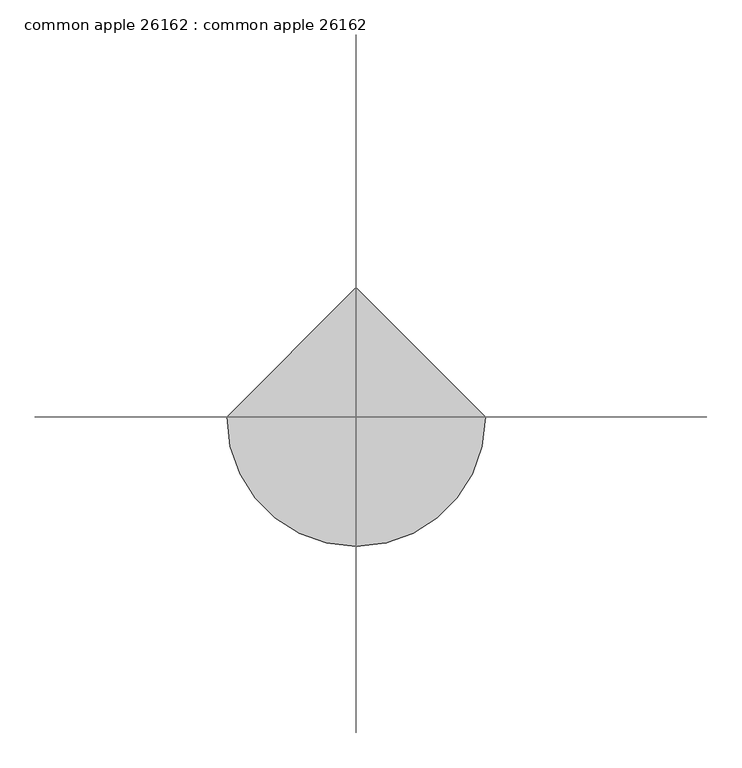
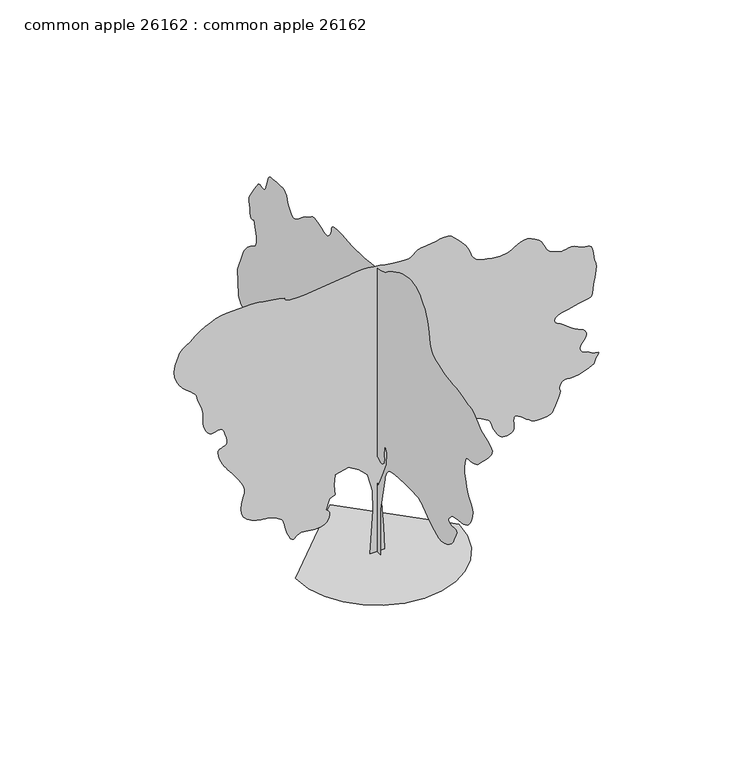
"""IFC4 building model written with IfcOpenShell, lengths in millimetres: proxy geometry, common apple 26162 : common apple 26162."""

from ifc_helpers import new_model, si_unit, origin, place, context, project, spatial, triangles, source, transform, mapped, element, save


def common_apple_26162_common_apple_26162_2cf08d23(model_context):
    return source(origin(), model_context, "Body", "Tessellation", [
        triangles([(-6.61e-05, -106.7031981, 0.0075972), (-6.25e-05, 141.1357166, 0.0075898), (-4.92e-05, 101.4814601, 465.9455781), (-3.19e-05, 131.2220957, 1031.0173004), (-1.83e-05, 230.3576144, 1437.4734501), (-8.7e-06, 398.8869896, 1675.3980263), (-1.1e-06, 587.2459139, 1834.016106), (2.7e-06, 765.6887283, 1873.6680462), (3.6e-06, 963.961219, 1804.2751888), (1.5e-06, 1023.4430534, 1705.1389435), (-4.1e-06, 904.4794573, 1576.2617809), (-8.5e-06, 944.1340136, 1407.7326782), (-1.46e-05, 1172.144878, 1090.4990622), (-1.49e-05, 1568.687534, 882.3128597), (-8.7e-06, 2143.6727863, 803.006436), (7.7e-06, 2490.6473923, 1179.7191977), (2.57e-05, 2847.5453751, 1606.0026981), (3.25e-05, 3402.6882339, 1556.4345028), (3.9e-05, 3600.9610153, 1675.3980263), (4.6e-05, 3591.0549339, 1913.3226025), (4.57e-05, 3412.6196045, 1992.6315697), (5.03e-05, 3283.7399712, 2210.7288677), (5.51e-05, 3591.0549339, 2220.6425068), (6.07e-05, 4205.6845688, 2101.6814541), (6.29e-05, 4275.3567696, 2137.8384041), (6.49e-05, 4342.3114037, 2174.2544952), (6.7e-05, 4403.9061905, 2211.1911942), (6.89e-05, 4457.4241447, 2248.9101128), (7.07e-05, 4500.1976967, 2287.6680668), (7.23e-05, 4529.5348595, 2327.7263775), (7.37e-05, 4542.7427742, 2369.3469475), (8.93e-05, 4572.4863075, 2874.9268433), (9.94e-05, 4403.9570595, 3301.215358), (0.0001002, 4386.5834106, 3334.8449913), (0.000101, 4360.9041641, 3374.6975006), (0.0001018, 4328.265168, 3418.5378479), (0.0001026, 4290.0887192, 3464.105706), (0.0001033, 4247.7471176, 3509.1651649), (0.0001039, 4202.636499, 3551.4561882), (0.0001043, 4156.1291634, 3588.718158), (0.0001045, 4111.323468, 3617.9027138), (0.0001046, 4070.8611122, 3640.1530998), (0.0001046, 4035.4281006, 3659.4571541), (0.0001048, 4005.7101471, 3679.8024239), (0.0001052, 3982.4182549, 3705.2026176), (0.000106, 3966.2384285, 3739.5941231), (0.0001073, 3957.8566727, 3786.9906487), (0.0001089, 3956.7898773, 3842.7945099), (0.0001107, 3961.4378494, 3899.6395866), (0.0001126, 3970.8614021, 3957.3738533), (0.0001145, 3984.0948967, 4015.7685448), (0.0001165, 4000.1982742, 4074.6966339), (0.0001185, 4018.2070587, 4133.9802246), (0.0001206, 4037.1553207, 4193.4417114), (0.0001203, 4062.5299347, 4172.9947037), (0.0001202, 4087.2188347, 4157.4244331), (0.0001204, 4110.5107269, 4151.5570587), (0.000121, 4131.7196068, 4160.2693176), (0.0001221, 4150.160051, 4188.3870781), (0.0001239, 4165.1460548, 4240.787368), (0.0001265, 4175.9410355, 4322.3213448), (0.000129, 4186.6092796, 4402.5600517), (0.0001308, 4198.1408432, 4455.5698975), (0.000132, 4205.3543564, 4492.9588943), (0.000133, 4202.9922913, 4526.3597626), (0.0001339, 4185.923275, 4567.406385), (0.0001352, 4148.8900703, 4627.7059021), (0.000137, 4086.736306, 4718.8666168), (0.0001389, 4019.8834099, 4816.9867905), (0.0001404, 3969.4896835, 4892.043837), (0.0001414, 3931.4405525, 4946.4759796), (0.0001421, 3901.5194138, 4982.6714447), (0.0001423, 3875.5858223, 5003.1184525), (0.0001421, 3849.5002052, 5010.2046478), (0.0001416, 3819.0709579, 5006.343837), (0.0001408, 3787.3208611, 4996.7176804), (0.0001401, 3759.4062859, 4987.6240494), (0.0001396, 3734.2601463, 4983.2045517), (0.0001394, 3710.841227, 4987.6240494), (0.0001396, 3688.1338921, 5005.0485672), (0.0001402, 3665.0704742, 5039.6435486), (0.0001416, 3640.6103394, 5095.574437), (0.0001432, 3619.2235634, 5160.9030075), (0.0001447, 3603.043737, 5219.9581238), (0.000146, 3587.5496246, 5271.4183548), (0.000147, 3568.2455704, 5313.8366959), (0.0001475, 3540.6103386, 5345.8661362), (0.0001475, 3500.1482735, 5366.109668), (0.0001469, 3442.3378487, 5373.1458664), (0.0001459, 3372.4368828, 5376.2445145), (0.0001451, 3300.6055115, 5383.3312912), (0.0001442, 3229.8412262, 5391.1034912), (0.0001434, 3163.0391991, 5396.2851517), (0.0001425, 3103.1713417, 5395.5485687), (0.0001414, 3053.2095657, 5385.642778), (0.0001402, 3016.0746231, 5363.2394943), (0.0001391, 2991.8429626, 5337.2044556), (0.0001382, 2976.4758774, 5316.3510773), (0.0001375, 2966.6462448, 5297.4283951), (0.0001368, 2959.0769394, 5277.1081238), (0.0001359, 2950.4664185, 5252.1148819), (0.0001348, 2937.5122673, 5219.1198029), (0.0001331, 2916.9382324, 5174.873085), (0.0001313, 2890.1666107, 5126.1051315), (0.0001296, 2860.6265533, 5083.2042618), (0.000128, 2827.9619774, 5048.4569641), (0.0001268, 2791.8432518, 5024.124147), (0.0001258, 2751.8890045, 5012.4399765), (0.0001253, 2707.794603, 5015.6909409), (0.0001252, 2659.1789658, 5036.0873703), (0.0001254, 2610.791803, 5068.0662323), (0.0001258, 2565.8846603, 5103.6768494), (0.0001263, 2521.8332794, 5141.7006912), (0.0001267, 2476.0523529, 5180.9436447), (0.0001272, 2425.9356445, 5220.212178), (0.0001274, 2368.8821503, 5258.2360199), (0.0001275, 2302.2908661, 5293.846637), (0.0001276, 2240.2945049, 5328.4671982), (0.0001279, 2193.5584042, 5362.0459625), (0.0001282, 2154.2798424, 5391.129071), (0.0001282, 2114.6558075, 5412.2365036), (0.0001278, 2066.8783459, 5421.8882401), (0.0001267, 2003.1496777, 5416.6304214), (0.0001247, 1915.6618492, 5392.9830276), (0.0001224, 1826.1497257, 5361.2837997), (0.0001207, 1757.9710384, 5335.9853439), (0.0001194, 1705.7434124, 5319.8816757), (0.0001187, 1664.0950825, 5315.7418121), (0.0001184, 1627.6484699, 5326.358606), (0.0001187, 1591.0293388, 5354.4766571), (0.0001195, 1548.8602558, 5402.8893997), (0.0001207, 1514.8419834, 5459.7853455), (0.000122, 1498.8602554, 5510.7630478), (0.0001232, 1489.8128426, 5554.806871), (0.0001241, 1476.6047825, 5590.874437), (0.0001244, 1448.1338459, 5617.9256927), (0.0001241, 1393.3079773, 5634.9182602), (0.0001229, 1301.0220406, 5640.8109238), (0.0001214, 1201.3955635, 5639.6935501), (0.0001202, 1126.7398006, 5636.6454803), (0.0001192, 1069.2519579, 5632.2259827), (0.0001184, 1021.1290958, 5626.9425842), (0.0001175, 974.5682751, 5621.3039749), (0.0001165, 921.7642307, 5615.8426804), (0.0001154, 854.9113346, 5611.0679718), (0.0001143, 784.7082069, 5608.019902), (0.0001133, 723.0014357, 5607.2071609), (0.0001125, 663.7228592, 5608.4768509), (0.0001116, 600.8019178, 5611.6516571), (0.0001107, 528.1680156, 5616.5792633), (0.0001096, 439.7556433, 5623.0567749), (0.0001082, 329.4941322, 5630.9051331), (0.0001067, 206.9466705, 5641.7254028), (0.0001053, 88.3885184, 5656.6861176), (0.0001042, -22.1921751, 5675.1262711), (0.0001034, -120.8075788, 5696.3354416), (0.0001029, -203.4686488, 5719.6276245), (0.0001027, -266.1871316, 5744.3162338), (0.0001028, -304.9729546, 5769.6908478), (0.0001032, -347.9523442, 5804.4381454), (0.0001036, -420.583703, 5853.4089935), (0.0001039, -514.8939712, 5910.1532043), (0.000104, -622.9024584, 5968.31884), (0.0001039, -736.6335978, 6021.4301331), (0.0001035, -848.1092062, 6063.1118912), (0.0001027, -949.3562239, 6086.9371811), (0.0001016, -1039.2697763, 6095.8017563), (0.0001004, -1122.4243664, 6096.0046509), (9.9e-05, -1199.3330441, 6086.1494385), (9.73e-05, -1270.5191059, 6064.8391113), (9.53e-05, -1336.5033051, 6030.7016602), (9.29e-05, -1397.8062492, 5982.3650757), (9.01e-05, -1454.9462208, 5918.407933), (8.77e-05, -1502.3755932, 5861.1056168), (8.62e-05, -1536.9730453, 5825.4944183), (8.5e-05, -1562.8963177, 5799.256485), (8.38e-05, -1584.313615, 5770.0716385), (8.22e-05, -1605.3828232, 5725.6220261), (7.96e-05, -1630.2698215, 5653.5874695), (7.58e-05, -1663.1323505, 5541.6751144), (7.16e-05, -1693.8258259, 5415.6147858), (6.81e-05, -1715.6747829, 5307.5626602), (6.5e-05, -1738.0446384, 5214.9799393), (6.21e-05, -1770.3000824, 5135.1981812), (5.93e-05, -1821.8062408, 5065.6530075), (5.62e-05, -1901.9230076, 5003.7532974), (5.28e-05, -2020.0178341, 4946.8823502), (4.95e-05, -2152.913356, 4902.7117905), (4.69e-05, -2273.494804, 4876.3974083), (4.48e-05, -2385.2295536, 4861.5384315), (4.29e-05, -2491.5921021, 4851.7340881), (4.1e-05, -2596.0345642, 4840.5071571), (3.89e-05, -2702.0542557, 4821.482737), (3.62e-05, -2813.1030006, 4788.2594742), (3.39e-05, -2912.3155495, 4758.5159409), (3.24e-05, -2986.585144, 4746.9843773), (3.14e-05, -3044.8780975, 4742.742485), (3.04e-05, -3096.2371719, 4734.8432579), (2.89e-05, -3149.6786774, 4712.3896866), (2.66e-05, -3214.2200867, 4664.4344742), (2.28e-05, -3298.878582, 4580.0809021), (1.85e-05, -3408.6320572, 4492.8062874), (1.5e-05, -3530.0185432, 4434.3354378), (1.2e-05, -3644.3188339, 4390.95233), (9.4e-06, -3732.7616913, 4348.9659393), (7.2e-06, -3776.6273277, 4294.6608238), (5.1e-06, -3757.196537, 4214.3459587), (3e-06, -3655.7486595, 4094.3056114), (1.1e-06, -3529.027906, 3968.7786804), (-3e-07, -3439.3912262, 3876.7287758), (-1.3e-06, -3376.6531952, 3811.5525215), (-1.9e-06, -3330.5522301, 3766.670668), (-2.3e-06, -3290.852037, 3735.479258), (-2.3e-06, -3247.3671913, 3711.4002045), (-2.2e-06, -3189.8108208, 3687.854258), (-1.7e-06, -3124.3802216, 3671.1919029), (-1e-06, -3064.487075, 3666.3404549), (-2e-07, -3010.8420937, 3664.4356293), (2e-07, -2964.1568619, 3656.6378494), (2e-07, -2925.0662247, 3634.0825401), (-8e-07, -2894.3070557, 3587.9559952), (-2.8e-06, -2872.5897766, 3509.3939301), (-5.1e-06, -2860.8041588, 3423.8465355), (-7.1e-06, -2858.3659355, 3357.9081184), (-8.8e-06, -2863.7507813, 3304.4410332), (-1.04e-05, -2875.358503, 3256.3335045), (-1.21e-05, -2891.6653564, 3206.498465), (-1.41e-05, -2911.070858, 3147.8244301), (-1.67e-05, -2932.0768433, 3073.199334), (-1.95e-05, -2961.2613991, 2993.8242371), (-2.22e-05, -3001.7234642, 2923.6186386), (-2.47e-05, -3046.5291595, 2859.6612053), (-2.72e-05, -3088.7187355, 2798.9806068), (-2.95e-05, -3121.3830208, 2738.6555099), (-3.16e-05, -3137.5628471, 2675.7398735), (-3.35e-05, -3130.349334, 2607.2612045), (-3.52e-05, -3109.3942177, 2540.281572), (-3.66e-05, -3087.7280983, 2482.819091), (-3.77e-05, -3063.4964378, 2433.5098915), (-3.85e-05, -3034.7182526, 2390.964814), (-3.91e-05, -2999.5645844, 2353.7970245), (-3.94e-05, -2956.0544495, 2320.6169277), (-3.96e-05, -2902.3333099, 2290.0378349), (-3.93e-05, -2836.3948929, 2266.2507694), (-3.86e-05, -2760.9314758, 2251.4832115), (-3.77e-05, -2680.9721123, 2241.3942924), (-3.68e-05, -2601.4955681, 2231.6559334), (-3.61e-05, -2527.6041481, 2217.9272655), (-3.58e-05, -2464.279525, 2195.8749779), (-3.62e-05, -2416.56049, 2161.1632885), (-3.68e-05, -2383.2356346, 2123.2410393), (-3.73e-05, -2359.9691769, 2093.2995529), (-3.79e-05, -2347.1065899, 2069.598674), (-3.84e-05, -2344.9984337, 2050.4090023), (-3.9e-05, -2353.9875652, 2033.9929985), (-3.98e-05, -2374.4217831, 2018.6158848), (-4.07e-05, -2406.646851, 2002.5452087), (-4.16e-05, -2449.8269188, 1993.9041664), (-4.23e-05, -2498.3841293, 1996.5330757), (-4.28e-05, -2545.5646797, 2002.2862129), (-4.34e-05, -2584.5791588, 2003.0075352), (-4.41e-05, -2608.6837921, 1990.5513187), (-4.52e-05, -2611.0967262, 1956.7642822), (-4.66e-05, -2585.0869766, 1893.4953243), (-4.83e-05, -2549.9080193, 1821.1814243), (-4.96e-05, -2524.6272949, 1762.91376), (-5.07e-05, -2502.1126808, 1714.5318295), (-5.16e-05, -2475.2625755, 1671.8725147), (-5.23e-05, -2436.9668026, 1630.7726978), (-5.27e-05, -2380.1140228, 1587.0720222), (-5.3e-05, -2297.5969666, 1536.6072247), (-5.28e-05, -2203.8378639, 1496.8968578), (-5.19e-05, -2116.842738, 1484.7582092), (-5.03e-05, -2034.8743401, 1494.9892708), (-4.83e-05, -1956.2028339, 1522.3883251), (-4.6e-05, -1879.090971, 1561.7532188), (-4.35e-05, -1801.803828, 1607.8822346), (-4.09e-05, -1722.6115688, 1655.5707481), (-3.83e-05, -1647.9584221, 1703.6352562), (-3.59e-05, -1583.013113, 1752.3931812), (-3.37e-05, -1524.1383636, 1798.8980461), (-3.16e-05, -1467.6919544, 1840.2010483), (-2.97e-05, -1410.0313751, 1873.3506237), (-2.82e-05, -1347.5167316, 1895.4053822), (-2.69e-05, -1276.503479, 1903.4089634), (-2.54e-05, -1177.6846561, 1904.2776604), (-2.33e-05, -1044.3574018, 1905.4916851), (-2.11e-05, -891.7820492, 1904.9710773), (-1.89e-05, -735.2163151, 1900.6352955), (-1.7e-05, -589.9230761, 1890.4040886), (-1.58e-05, -471.1627742, 1872.1948803), (-1.55e-05, -394.1956335, 1843.9297451), (-1.6e-05, -348.7041879, 1805.3140789), (-1.68e-05, -313.0958962, 1758.377409), (-1.8e-05, -285.7248199, 1704.5039532), (-1.95e-05, -264.9450744, 1645.0805454), (-2.11e-05, -249.1058704, 1581.494165), (-2.29e-05, -236.5620685, 1515.1341167), (-2.48e-05, -225.6659676, 1447.3870892), (-3.91e-05, -116.6168281, 912.0537769), (-2.05e-05, -27.3946828, 1318.5099266), (-1.32e-05, -176.0980811, 1635.74347), (-6.6e-06, -304.975498, 1923.2362415), (2e-07, -324.8002327, 2161.1632885), (4.8e-06, -255.4073572, 2280.1241959), (-4e-07, -225.6657133, 2091.767815), (-1.7e-06, -231.7353101, 2049.4539734), (-3e-06, -235.984215, 2008.1814926), (-4.2e-06, -236.5910275, 1968.9892628), (-5.2e-06, -231.7353101, 1932.9186447), (-6e-06, -219.5961346, 1901.0111446), (-6.5e-06, -198.3530817, 1874.3056526), (-6.6e-06, -166.1844602, 1853.8433842), (-6.2e-06, -129.2182845, 1848.5829494), (-5.3e-06, -95.0268123, 1860.3152275), (-4.3e-06, -63.9562343, 1879.3348515), (-3.4e-06, -36.354542, 1895.9235191), (-2.9e-06, -12.5678035, 1900.3761543), (-3.1e-06, 7.0569383, 1882.9772163), (-4.4e-06, 22.1729471, 1834.016106), (-6.1e-06, 32.8958209, 1768.9260384), (-7.8e-06, 39.9768386, 1709.0403042), (-9.4e-06, 44.0233167, 1653.4904972), (-1.1e-05, 45.6418044, 1601.4077751), (-1.24e-05, 45.4396183, 1551.9260571), (-1.39e-05, 44.0233167, 1504.1789715), (-1.53e-05, 41.9999482, 1457.3007282), (139.590126, 0.0003305, 0.0), (-135.4471285, 0.0003387, 0.0), (-74.3278259, 0.000241, 845.4879272), (-84.5142454, 0.0002472, 1242.76455), (-186.3807747, 0.0002013, 1599.294532), (-339.1791879, 0.0002082, 1752.0933449), (-542.9102117, 0.000216, 1874.3335579), (-797.5758808, 0.0002227, 1813.2134514), (-817.9492012, 0.0002203, 1609.4824276), (-797.5758808, 0.0002168, 1415.9368286), (-899.4426281, 0.0002191, 1365.0021469), (-970.7481594, 0.0002183, 1171.4565479), (-951.3247084, 0.0002718, 1158.1240768), (-933.2373676, 0.000271, 1143.3616058), (-917.8246456, 0.0002703, 1125.7517796), (-906.4200365, 0.0002696, 1103.8645981), (-900.3621214, 0.000269, 1076.2750757), (-900.9870106, 0.0002686, 1041.555756), (-909.6280529, 0.0002682, 998.2868128), (-928.5764603, 0.0002681, 955.1042742), (-957.6798437, 0.0002684, 921.0098436), (-994.6267164, 0.0002692, 895.1144766), (-1037.0955631, 0.0002701, 876.5217161), (-1082.7698101, 0.0002713, 864.3449158), (-1129.3382612, 0.0002726, 857.6926329), (-1174.4791832, 0.0002739, 855.6733521), (-1218.6700905, 0.0002753, 858.4063974), (-1263.5747623, 0.0002767, 865.0586803), (-1308.6573303, 0.0002782, 873.3161705), (-1353.3816353, 0.0002796, 880.857498), (-1397.217041, 0.000281, 885.3710306), (-1439.6273884, 0.0002823, 884.5404854), (-1480.0769543, 0.0002833, 876.0466724), (-1514.854628, 0.0002841, 857.900905), (-1542.5051205, 0.0002846, 834.4084436), (-1565.8782578, 0.000285, 812.6990856), (-1587.8238659, 0.0002854, 799.9000122), (-1611.1970032, 0.0002862, 803.1359339), (-1638.8473503, 0.0002874, 829.5392641), (-1673.6225533, 0.000235, 886.2346407), (-1706.6171963, 0.0002371, 959.4984827), (-1729.2790398, 0.0002388, 1029.5593225), (-1744.988982, 0.0002402, 1094.4487484), (-1757.1353336, 0.0002415, 1152.2135365), (-1769.1037891, 0.0002426, 1200.8900711), (-1784.2803337, 0.0002436, 1238.5177162), (-1806.0481911, 0.0002446, 1263.1378704), (-1833.1626698, 0.0002457, 1282.7670502), (-1863.3073414, 0.0002469, 1305.4288937), (-1898.2629112, 0.0002483, 1329.1576778), (-1939.8122646, 0.0002499, 1351.9948013), (-1989.7334908, 0.0002517, 1371.9820988), (-2049.8147072, 0.0002537, 1387.1586433), (-2121.8338577, 0.000256, 1395.5635082), (-2205.4938675, 0.0002044, 1404.6210949), (-2294.67854, 0.0002073, 1424.3695988), (-2382.4381542, 0.0002104, 1456.7724174), (-2461.8232796, 0.0002135, 1503.7853909), (-2525.8821602, 0.0002163, 1567.3691551), (-2567.6627495, 0.0002188, 1649.4849277), (-2580.2355286, 0.0002207, 1752.0933449), (-2568.9835991, 0.0002218, 1851.4048702), (-2548.8159348, 0.0002224, 1927.9097935), (-2527.0379036, 0.0002227, 1989.979842), (-2510.9723145, 0.0001688, 2045.9893593), (-2507.9117455, 0.0001695, 2104.3180664), (-2525.1659248, 0.0001711, 2173.3375454), (-2570.0503944, 0.0001737, 2261.4222851), (-2629.7912247, 0.0001769, 2355.7756828), (-2686.3316689, 0.0001798, 2438.7243988), (-2738.9604332, 0.0001825, 2511.3356644), (-2786.9665146, 0.0001849, 2574.6730774), (-2829.6130394, 0.0001327, 2629.841803), (-2866.1890045, 0.0001345, 2677.8478844), (-2896.008696, 0.000136, 2719.8086952), (-2924.6092758, 0.0001376, 2767.4084061), (-2955.1652596, 0.0001394, 2827.2762634), (-2983.4100471, 0.0001412, 2893.0114952), (-3005.0764572, 0.0001428, 2958.2389091), (-3015.8461487, 0.000144, 3016.5062828), (-3011.4772293, 0.0001446, 3061.4137161), (-2987.7028084, 0.0001442, 3086.5342758), (-2951.4823448, 0.0001433, 3098.8532913), (-2915.109565, 0.0001425, 3111.5533882), (-2882.1147766, 0.0001417, 3127.4282913), (-2856.0800285, 0.0001413, 3149.3740448), (-2840.5350471, 0.0001413, 3180.2349518), (-2839.0871704, 0.0001418, 3222.8561874), (-2855.2669968, 0.0001432, 3280.0823456), (-2877.0348541, 9.05e-05, 3338.9342766), (-2892.2240433, 9.16e-05, 3385.5177704), (-2904.1875572, 9.25e-05, 3421.2048363), (-2916.3286766, 9.32e-05, 3447.4686401), (-2932.0259743, 9.4e-05, 3465.705899), (-2954.70802, 9.48e-05, 3477.3389099), (-2987.7028084, 9.59e-05, 3483.8161308), (-3026.4123642, 9.7e-05, 3481.8857254), (-3064.2583099, 9.8e-05, 3472.1066711), (-3101.5455688, 9.9e-05, 3461.6419029), (-3138.6805115, 0.0001, 3457.552327), (-3175.9930595, 0.0001013, 3467.026458), (-3213.8137161, 0.0001029, 3497.1763618), (-3252.5488518, 0.0001049, 3555.1138138), (-3281.1747208, 0.0001068, 3626.7419998), (-3293.239682, 0.0001082, 3695.3474052), (-3295.8558014, 0.0001093, 3764.1307068), (-3296.1351448, 0.0001104, 3836.3175797), (-3301.2406471, 5.74e-05, 3915.0575409), (-3318.2840836, 5.93e-05, 4003.6274254), (-3354.4028091, 6.19e-05, 4105.2020393), (-3391.2836975, 6.43e-05, 4197.0231789), (-3411.2481766, 6.59e-05, 4259.8120789), (-3422.2972115, 6.68e-05, 4301.925206), (-3432.4570564, 6.76e-05, 4331.7448975), (-3449.7545471, 6.85e-05, 4357.6276199), (-3482.1650688, 6.99e-05, 4387.9804184), (-3537.7657448, 7.22e-05, 4431.1606316), (-3609.6985634, 2.09e-05, 4488.5646858), (-3681.631382, 2.41e-05, 4556.1285851), (-3747.3157448, 2.72e-05, 4634.0305161), (-3800.5287758, 3.01e-05, 4722.4480843), (-3835.047599, 3.26e-05, 4821.5588951), (-3844.6231773, 3.45e-05, 4931.5152649), (-3822.9823471, 3.57e-05, 5052.5468307), (-3789.555899, -1.8e-05, 5157.9310959), (-3763.7749146, -1.77e-05, 5228.187854), (-3739.5941231, -1.77e-05, 5274.3902664), (-3710.9682541, -1.81e-05, 5307.5882401), (-3671.8270386, -1.88e-05, 5338.8555176), (-3616.1246246, -1.98e-05, 5379.1652664), (-3537.7657448, -2.13e-05, 5439.6429703), (-3445.4364967, -2.3e-05, 5511.6775269), (-3351.6849518, -2.48e-05, 5578.225209), (-3256.3079247, -2.67e-05, 5637.4326416), (-3159.1783882, -2.89e-05, 5687.5726044), (-3060.0675774, -3.12e-05, 5726.8155579), (-2958.8228851, -3.39e-05, 5753.4348633), (-2855.2669968, -3.68e-05, 5765.6015625), (-2376.4970924, -5.09e-05, 5775.7869873), (-2309.7356152, -5.29e-05, 5773.1197083), (-2232.8167637, -5.53e-05, 5765.6521408), (-2147.4320045, -3.8e-06, 5754.1458664), (-2055.2781818, -6.7e-06, 5739.4392059), (-1958.0469074, -9.9e-06, 5722.3449005), (-1857.4273224, -1.32e-05, 5703.6251129), (-1755.1159801, -1.65e-05, 5684.1181641), (-1751.9080364, -1.69e-05, 5664.6617935), (-1742.5530842, -1.75e-05, 5646.3739563), (-1720.9022255, -1.83e-05, 5630.3970245), (-1680.8107773, -1.97e-05, 5617.9001129), (-1616.1270802, -2.18e-05, 5610.0261749), (-1520.7042709, -2.46e-05, 5607.9437439), (-1388.3981026, -2.85e-05, 5612.8201904), (-614.2181774, -5.02e-05, 5704.4890137), (-538.3076946, -5.24e-05, 5711.4996323), (-472.1990845, 1e-07, 5721.8879517), (-409.4762778, -1.6e-06, 5732.8355392), (-343.7232419, -3.5e-06, 5741.4460602), (-268.5264692, -5.7e-06, 5744.8749207), (-177.4707081, -8.5e-06, 5740.3031067), (-64.1414019, -1.21e-05, 5724.8598633), (54.7118994, -1.59e-05, 5704.3111176), (159.4882483, -1.93e-05, 5686.4296509), (252.3260954, -2.23e-05, 5671.4183578), (335.3640864, -2.49e-05, 5659.4039749), (410.7386644, -2.73e-05, 5650.6155579), (480.5886887, -2.95e-05, 5645.205423), (547.0529457, -3.15e-05, 5643.3764648), (603.2428662, -3.3e-05, 5651.8346695), (646.0698669, -3.4e-05, 5673.6531052), (683.3697704, -3.47e-05, 5703.4983765), (722.9887184, -3.54e-05, 5736.0359253), (772.7625698, -3.64e-05, 5765.8806152), (840.5349592, -3.81e-05, 5787.6996323), (934.1441437, -4.07e-05, 5796.1828354), (1035.6832947, -4.37e-05, 5802.989978), (1124.0372766, -4.61e-05, 5818.3826431), (1202.2337391, -4.82e-05, 5834.6642075), (1273.3004768, -5.01e-05, 5844.1636276), (1340.2726971, -5.22e-05, 5839.2360214), (1406.173035, -5.46e-05, 5812.2103455), (1474.0342999, -3.2e-06, 5755.4161377), (1539.0152172, -6.2e-06, 5686.9627579), (1594.7301304, -8.7e-06, 5628.1366974), (1641.8903332, -1.09e-05, 5576.0666199), (1681.2120609, -1.28e-05, 5527.9335114), (1713.4041367, -1.44e-05, 5480.8671982), (1739.182505, -1.59e-05, 5431.9975067), (1759.2587505, -1.73e-05, 5378.5304214), (1777.3156425, -1.87e-05, 5324.8604416), (1798.9361252, -2e-05, 5277.2604401), (1827.6839344, -2.15e-05, 5235.5281036), (1867.1225155, 3.1e-05, 5199.4855362), (1920.8180752, 2.9e-05, 5169.0060013), (1992.3318787, 2.65e-05, 5143.8342819), (2085.229842, 2.34e-05, 5123.844223), (2181.6306438, 2.03e-05, 5109.4171967), (2262.7075264, 1.78e-05, 5100.6799393), (2330.5991673, 1.57e-05, 5097.123761), (2387.4419186, 1.4e-05, 5098.1905563), (2435.3767834, 1.27e-05, 5103.3722168), (2476.5374977, 1.16e-05, 5112.0844757), (2513.0678261, 1.07e-05, 5123.844223), (2552.2195061, 9.8e-06, 5144.4947067), (2599.1840813, 8.9e-06, 5175.4829315), (2653.1336952, 7.8e-06, 5209.6459625), (2713.1032906, 6.4e-06, 5239.9226028), (2778.2795448, 4.8e-06, 5259.1249191), (2847.697982, 2.7e-06, 5260.1661346), (2920.5196999, 2e-07, 5235.9094757), (2984.2992371, -2.2e-06, 5202.1528152), (3030.2478859, -4e-06, 5176.5747253), (3062.9883293, -5.3e-06, 5154.908606), (3087.1947006, -6.3e-06, 5132.9122742), (3107.4893921, -7.3e-06, 5106.2679703), (3128.4697975, -8.5e-06, 5070.73293), (3154.8094688, -1e-05, 5021.9905563), (3182.8510712, 4.27e-05, 4971.0890121), (3208.2256851, 4.13e-05, 4930.3473129), (3234.4639091, 4e-05, 4897.4289734), (3265.1724998, 3.87e-05, 4870.0475052), (3303.9076355, 3.72e-05, 4845.8667137), (3354.2252037, 3.53e-05, 4822.6004013), (3419.6808014, 3.3e-05, 4797.8859215), (3486.0258797, 3.08e-05, 4782.8237595), (3540.0769409, 2.92e-05, 4784.7032959), (3586.9909378, 2.8e-05, 4795.4729874), (3631.9489494, 2.68e-05, 4807.1571579), (3680.1326363, 2.55e-05, 4811.7036827), (3736.6730804, 2.36e-05, 4801.0863075), (3806.7519424, 2.1e-05, 4767.3299377), (3879.2181587, 1.84e-05, 4732.9890106), (3939.9240463, 1.63e-05, 4718.4346664), (3989.5811897, 1.48e-05, 4712.2626595), (4028.9003014, 1.35e-05, 4703.0678719), (4058.6185455, 1.22e-05, 4679.4204781), (4079.3957657, 6.51e-05, 4629.9412308), (4091.9941246, 6.34e-05, 4543.2253029), (4103.8306114, 6.18e-05, 4454.6301292), (4119.4261711, 6.04e-05, 4397.0481789), (4135.0217308, 5.94e-05, 4355.3161331), (4146.8835068, 5.84e-05, 4314.2950905), (4151.2268463, 5.74e-05, 4258.8467308), (4144.3688347, 5.64e-05, 4173.8330246), (4122.550399, 5.51e-05, 4044.0642014), (4100.096537, 0.000108, 3908.7329269), (4088.8698967, 0.0001069, 3812.0603394), (4081.3767494, 0.0001061, 3746.5791618), (4070.1501091, 0.0001058, 3704.7962471), (4047.6965378, 0.0001061, 3679.2184479), (4006.548468, 0.0001071, 3662.4034859), (3939.1874634, 0.0001089, 3646.8079262), (3844.4708611, 0.0001114, 3628.5706673), (3734.0822502, 0.0001144, 3608.1998177), (3619.7822502, 0.0001175, 3584.781189), (3513.3053192, 0.0001202, 3557.4761696), (3426.4373657, 0.0001224, 3525.3449913), (3370.9384277, 0.0001234, 3487.4990456), (3358.5429634, 0.0001231, 3443.0744316), (3371.5224037, 0.0001222, 3405.6092766), (3386.2799332, 0.0001214, 3384.1972115), (3405.8633308, 0.0001207, 3371.1669022), (3433.2700882, 0.0001197, 3358.8478867), (3471.5476936, 0.0001182, 3339.5694122), (3523.7447983, 0.0001162, 3305.6857246), (3592.8327324, 0.0001133, 3249.5260712), (3669.2870773, 0.0001101, 3189.9884262), (3740.381575, 0.0001074, 3147.3671906), (3804.5419029, 0.000105, 3116.150782), (3860.1425789, 0.0001572, 3090.8014572), (3905.55783, 0.0001555, 3065.8332138), (3939.2383324, 0.000154, 3035.6833099), (3959.558313, 0.0001528, 2994.8654526), (3960.2948959, 0.0001521, 2946.884951), (3941.8038734, 0.0001519, 2899.2852402), (3912.2635254, 0.0001521, 2852.3968231), (3879.8530037, 0.0001524, 2806.5752014), (3852.8020386, 0.0001525, 2762.1758766), (3839.2892006, 0.0001523, 2719.554641), (3847.5189308, 0.0001514, 2679.0672867), (3870.582058, 0.0001503, 2647.1645828), (3896.1598572, 0.0001492, 2627.2256836), (3924.2270393, 0.0001482, 2614.9319572), (3954.7830231, 0.0001472, 2606.0168037), (3987.8286804, 0.000146, 2596.2121696), (4023.3887192, 0.0001447, 2581.2517456), (4061.4378502, 0.0001432, 2556.842189), (4100.7569618, 0.0001417, 2534.5891869), (4137.7648773, 0.0001405, 2524.8203064), (4168.8798386, 0.0001395, 2521.2847664), (4190.5462486, 0.0001388, 2517.7515518), (4199.2329277, 0.0001384, 2507.9803459), (4191.3334099, 0.0001926, 2485.7375175), (4163.2918076, 0.0001928, 2444.7824593), (4135.3263634, 0.0001929, 2399.7888393), (4122.8550316, 0.0001928, 2366.7332989), (4115.1842789, 0.0001927, 2341.3408081), (4101.6461517, 0.0001927, 2319.3343025), (4071.521537, 0.0001933, 2296.4387524), (4014.1430626, 0.0001946, 2268.3717155), (3918.8166138, 0.0001969, 2230.8633945), (3811.1205711, 0.0001996, 2200.6297749), (3722.1443161, 0.0002021, 2191.0666958), (3649.3987564, 0.0002043, 2192.9081532), (3590.3436401, 0.0002062, 2196.8884335), (3542.540744, 0.0002075, 2193.7413872), (3503.4501068, 0.0002084, 2174.1985394), (3470.6079254, 0.0002087, 2128.9966473), (3451.2532928, 0.0002086, 2081.7474964), (3449.1702805, 0.0002083, 2055.3443115), (3456.7142967, 0.0002078, 2039.4564732), (3466.2137169, 0.0002073, 2023.7466763), (3470.0236588, 0.0002068, 1997.8792145), (3460.4480804, 0.0002064, 1951.5191082), (3429.8662262, 0.0002061, 1874.3335579), (3393.2393921, 0.0002059, 1787.376511), (3366.4171921, 0.0002057, 1717.5239433), (3342.9982727, 0.0002056, 1663.1755165), (3316.5315742, 0.0002058, 1622.7259506), (3280.6157433, 0.0002064, 1594.5725819), (3228.850589, 0.0002077, 1577.1101303), (3154.8094688, 0.0002098, 1568.7357868), (3080.6413216, 0.0002119, 1565.2609989), (3027.8349518, 0.0002135, 1564.6361824), (2989.0998161, 0.0002147, 1568.469088), (2957.146534, 0.0002158, 1578.3572926), (2924.6598541, 0.000217, 1595.9086922), (2884.3248161, 0.0002186, 1622.7259506), (2828.8511673, 0.0002209, 1660.4146385), (2768.830703, 0.0002233, 1702.4363468), (2719.1482704, 0.0002253, 1739.6499184), (2678.9146797, 0.000227, 1769.7336926), (2647.2154518, 0.0002282, 1790.3763279), (2623.1869766, 0.0002291, 1799.2561638), (2605.9403549, 0.0002295, 1794.0567719), (2594.5613983, 0.0002295, 1772.4668106), (2588.1350464, 0.0002293, 1744.7273701), (2585.6459541, 0.000229, 1721.445797), (2586.0014557, 0.0002287, 1700.833683), (2588.1350464, 0.0002283, 1681.1130844), (2591.00522, 0.0002279, 1660.5034412), (2593.494603, 0.0002275, 1637.219252), (2594.5613983, 0.0002271, 1609.4824276), (2593.1135216, 0.0002267, 1579.0989624), (2587.906572, 0.0002264, 1549.7873795), (2577.7211472, 0.0002263, 1522.6143288), (2561.2872665, 0.0002264, 1498.6468964), (2537.3884346, 0.0002268, 1478.9568192), (2504.7494385, 0.0002276, 1464.6108925), (2462.1331444, 0.0002288, 1456.6836147), (2418.7144283, 0.00023, 1454.9893867), (2382.9562912, 0.0002312, 1459.35569), (2352.5447754, 0.0002322, 1470.8491745), (2325.1635979, 0.0002333, 1490.5392517), (2298.4935688, 0.0002346, 1519.4951878), (2270.2207306, 0.000236, 1558.7865395), (2238.0288002, 0.0002377, 1609.4824276), (2208.2396301, 0.0002394, 1664.8392231), (2186.8274197, 0.0001866, 1716.8127949), (2170.9397266, 0.0001878, 1764.5088661), (2157.7241089, 0.0001888, 1807.0362122), (2144.3307404, 0.0001897, 1843.5054977), (2127.9070335, 0.0001907, 1873.0254982), (2105.6033077, 0.0001917, 1894.7068783), (2074.6583942, 0.0001929, 1913.6528149), (2035.1589157, 0.0001944, 1935.2732975), (1988.5319653, 0.0001961, 1959.1214058), (1936.2028919, 0.0001981, 1984.7525448), (1879.5964634, 0.0002001, 2011.717178), (1820.1400635, 0.0002023, 2039.5759426), (1759.2587505, 0.0002046, 2067.8791569), (1412.9141933, 0.0002149, 2067.8791569), (1219.3685944, 0.0002173, 1843.7721966), (1214.8270838, 0.000217, 1813.2134514), (1209.2136909, 0.0002167, 1782.6522354), (1201.4616205, 0.0002165, 1752.0933449), (1190.5040045, 0.0002164, 1721.5345997), (1175.2665625, 0.0002164, 1690.9733837), (1154.6874407, 0.0002165, 1660.4146385), (1127.6898153, 0.0002169, 1629.855748), (1103.6638836, 0.0002172, 1604.0163368), (1088.903956, 0.0002174, 1586.5538853), (1077.7076191, 0.0002175, 1575.8629681), (1064.3726046, 0.0002179, 1570.3384506), (1043.1966442, 0.0002185, 1568.3775238), (1008.4798679, 0.0002195, 1568.3775238), (954.5175367, 0.0002211, 1568.7357868), (886.9839409, 0.0002232, 1571.6161343), (817.1339167, 0.0002254, 1579.3072346), (747.6394667, 0.0002276, 1590.3841747), (681.1726662, 0.0002298, 1603.4220417), (620.41075, 0.0002318, 1616.9957771), (568.0206702, 0.0002335, 1629.6755264), (526.6821324, 0.0002349, 1640.0411728), (491.1627162, 0.0002361, 1650.5543392), (454.5739975, 0.0002374, 1664.275304), (417.0937271, 0.0002388, 1680.6684895), (378.9022719, 0.0002402, 1699.2003525), (340.1748393, 0.0001874, 1719.3350246), (301.0918324, 0.0001889, 1740.5414337), (261.828495, 0.0001904, 1762.2813858), (78.4708189, 0.0002443, 1375.1901878), (68.2843994, 0.0002402, 1079.7776962), (119.217278, 0.0002837, 458.3966929), (-1547.0796959, 1.1e-06, 0.0099807), (-1506.1805935, -354.4877738, 0.0099913), (-1389.6986046, -680.02964, 0.010001), (-1206.9607035, -967.2962626, 0.0100095), (-967.2962626, -1206.9607035, 0.0100167), (-680.02964, -1389.6986046, 0.0100221), (-354.4877738, -1506.1805935, 0.0100256), (6.76e-05, -1547.0796959, 0.0100268), (354.4877738, -1506.1805935, 0.0100256), (680.02964, -1389.6986046, 0.0100221), (967.2962626, -1206.9607035, 0.0100167), (1206.9607035, -967.2962626, 0.0100095), (1389.6986046, -680.02964, 0.010001), (1506.1805935, -354.4877738, 0.0099913), (1547.0796959, 0.0001258, 0.0099807), (-0.0002029, 1547.0796959, 0.0099346)], [[300, 1, 301], [299, 300, 301], [299, 301, 302], [298, 299, 302], [297, 298, 302], [296, 297, 302], [296, 302, 303], [295, 296, 303], [294, 295, 303], [293, 294, 303], [292, 293, 303], [1, 2, 3], [301, 1, 3], [301, 3, 4], [301, 4, 5], [327, 301, 5], [326, 327, 5], [326, 5, 6], [325, 326, 6], [324, 325, 6], [323, 324, 6], [322, 323, 6], [321, 322, 6], [320, 321, 6], [19, 20, 21], [18, 19, 21], [17, 18, 21], [17, 21, 22], [320, 6, 7], [319, 320, 7], [291, 292, 303], [291, 303, 304], [290, 291, 304], [261, 262, 263], [260, 261, 263], [260, 263, 264], [259, 260, 264], [259, 264, 265], [258, 259, 265], [10, 11, 12], [14, 15, 16], [258, 265, 266], [257, 258, 266], [205, 206, 207], [204, 205, 207], [204, 207, 208], [203, 204, 208], [203, 208, 209], [202, 203, 209], [202, 209, 210], [257, 266, 267], [10, 12, 13], [257, 267, 268], [257, 268, 269], [256, 257, 269], [256, 269, 270], [256, 270, 271], [255, 256, 271], [255, 271, 272], [255, 272, 273], [255, 273, 274], [255, 274, 275], [255, 275, 276], [255, 276, 277], [254, 255, 277], [254, 277, 278], [254, 278, 279], [254, 279, 280], [253, 254, 280], [253, 280, 281], [253, 281, 282], [289, 290, 304], [10, 13, 14], [10, 14, 16], [10, 16, 17], [10, 17, 22], [9, 10, 22], [201, 202, 210], [201, 210, 211], [201, 211, 212], [201, 212, 213], [201, 213, 214], [201, 214, 215], [201, 215, 216], [201, 216, 217], [201, 217, 218], [201, 218, 219], [200, 201, 219], [199, 200, 219], [198, 199, 219], [197, 198, 219], [196, 197, 219], [195, 196, 219], [194, 195, 219], [194, 219, 220], [193, 194, 220], [192, 193, 220], [191, 192, 220], [190, 191, 220], [189, 190, 220], [189, 220, 221], [188, 189, 221], [252, 253, 282], [252, 282, 283], [188, 221, 222], [187, 188, 222], [251, 252, 283], [187, 222, 223], [23, 24, 25], [318, 319, 7], [56, 57, 58], [56, 58, 59], [55, 56, 59], [55, 59, 60], [54, 55, 60], [54, 60, 61], [54, 61, 62], [23, 25, 26], [186, 187, 223], [23, 26, 27], [23, 27, 28], [23, 28, 29], [23, 29, 30], [23, 30, 31], [23, 31, 32], [23, 32, 33], [23, 33, 34], [23, 34, 35], [23, 35, 36], [23, 36, 37], [23, 37, 38], [23, 38, 39], [23, 39, 40], [23, 40, 41], [23, 41, 42], [23, 42, 43], [23, 43, 44], [22, 23, 44], [22, 44, 45], [9, 22, 45], [9, 45, 46], [9, 46, 47], [9, 47, 48], [8, 9, 48], [8, 48, 49], [8, 49, 50], [8, 50, 51], [8, 51, 52], [8, 52, 53], [8, 53, 54], [250, 251, 283], [250, 283, 284], [288, 289, 304], [288, 304, 305], [186, 223, 224], [287, 288, 305], [313, 314, 315], [312, 313, 315], [311, 312, 315], [310, 311, 315], [310, 315, 316], [309, 310, 316], [308, 309, 316], [308, 316, 317], [307, 308, 317], [306, 307, 317], [306, 317, 318], [305, 306, 318], [305, 318, 7], [305, 7, 8], [305, 8, 54], [305, 54, 62], [305, 62, 63], [305, 63, 64], [305, 64, 65], [305, 65, 66], [305, 66, 67], [305, 67, 68], [305, 68, 69], [305, 69, 70], [305, 70, 71], [305, 71, 72], [305, 72, 73], [305, 73, 74], [305, 74, 75], [305, 75, 76], [305, 76, 77], [305, 77, 78], [305, 78, 79], [305, 79, 80], [305, 80, 81], [305, 81, 82], [305, 82, 83], [305, 83, 84], [305, 84, 85], [305, 85, 86], [305, 86, 87], [305, 87, 88], [305, 88, 89], [305, 89, 90], [305, 90, 91], [305, 91, 92], [134, 135, 136], [134, 136, 137], [133, 134, 137], [133, 137, 138], [132, 133, 138], [132, 138, 139], [132, 139, 140], [131, 132, 140], [131, 140, 141], [131, 141, 142], [131, 142, 143], [130, 131, 143], [130, 143, 144], [130, 144, 145], [286, 287, 305], [186, 224, 225], [185, 186, 225], [249, 250, 284], [130, 145, 146], [285, 286, 305], [249, 284, 285], [249, 285, 305], [248, 249, 305], [234, 235, 236], [233, 234, 236], [233, 236, 237], [232, 233, 237], [232, 237, 238], [232, 238, 239], [232, 239, 240], [232, 240, 241], [232, 241, 242], [232, 242, 243], [232, 243, 244], [232, 244, 245], [231, 232, 245], [231, 245, 246], [231, 246, 247], [230, 231, 247], [230, 247, 248], [230, 248, 305], [229, 230, 305], [228, 229, 305], [227, 228, 305], [226, 227, 305], [225, 226, 305], [185, 225, 305], [184, 185, 305], [183, 184, 305], [182, 183, 305], [181, 182, 305], [180, 181, 305], [179, 180, 305], [178, 179, 305], [177, 178, 305], [176, 177, 305], [175, 176, 305], [174, 175, 305], [173, 174, 305], [172, 173, 305], [171, 172, 305], [170, 171, 305], [169, 170, 305], [168, 169, 305], [167, 168, 305], [166, 167, 305], [165, 166, 305], [164, 165, 305], [163, 164, 305], [162, 163, 305], [161, 162, 305], [160, 161, 305], [159, 160, 305], [158, 159, 305], [157, 158, 305], [156, 157, 305], [155, 156, 305], [154, 155, 305], [153, 154, 305], [152, 153, 305], [151, 152, 305], [150, 151, 305], [149, 150, 305], [148, 149, 305], [147, 148, 305], [146, 147, 305], [130, 146, 305], [129, 130, 305], [128, 129, 305], [127, 128, 305], [126, 127, 305], [125, 126, 305], [124, 125, 305], [123, 124, 305], [122, 123, 305], [121, 122, 305], [120, 121, 305], [119, 120, 305], [118, 119, 305], [117, 118, 305], [116, 117, 305], [115, 116, 305], [114, 115, 305], [113, 114, 305], [112, 113, 305], [111, 112, 305], [110, 111, 305], [109, 110, 305], [108, 109, 305], [107, 108, 305], [94, 95, 96], [94, 96, 97], [93, 94, 97], [93, 97, 98], [93, 98, 99], [93, 99, 100], [93, 100, 101], [92, 93, 101], [92, 101, 102], [92, 102, 103], [92, 103, 104], [92, 104, 105], [106, 107, 305], [106, 305, 92], [106, 92, 105], [328, 329, 330], [731, 328, 330], [730, 731, 330], [730, 330, 331], [729, 730, 331], [729, 331, 332], [728, 729, 332], [472, 473, 474], [336, 337, 338], [728, 332, 333], [618, 619, 620], [617, 618, 620], [617, 620, 621], [616, 617, 621], [615, 616, 621], [615, 621, 622], [614, 615, 622], [614, 622, 623], [472, 474, 475], [613, 614, 623], [612, 613, 623], [612, 623, 624], [612, 624, 625], [612, 625, 626], [612, 626, 627], [612, 627, 628], [611, 612, 628], [610, 611, 628], [610, 628, 629], [609, 610, 629], [609, 629, 630], [608, 609, 630], [608, 630, 631], [608, 631, 632], [607, 608, 632], [607, 632, 633], [606, 607, 633], [363, 364, 365], [363, 365, 366], [362, 363, 366], [362, 366, 367], [361, 362, 367], [361, 367, 368], [360, 361, 368], [360, 368, 369], [360, 369, 370], [359, 360, 370], [359, 370, 371], [358, 359, 371], [358, 371, 372], [407, 408, 409], [407, 409, 410], [406, 407, 410], [406, 410, 411], [405, 406, 411], [405, 411, 412], [404, 405, 412], [403, 404, 412], [403, 412, 413], [402, 403, 413], [401, 402, 413], [400, 401, 413], [399, 400, 413], [357, 358, 372], [606, 633, 634], [399, 413, 414], [398, 399, 414], [728, 333, 334], [357, 372, 373], [356, 357, 373], [562, 563, 564], [561, 562, 564], [561, 564, 565], [560, 561, 565], [559, 560, 565], [559, 565, 566], [397, 398, 414], [355, 356, 373], [354, 355, 373], [353, 354, 373], [352, 353, 373], [351, 352, 373], [350, 351, 373], [349, 350, 373], [348, 349, 373], [347, 348, 373], [346, 347, 373], [345, 346, 373], [344, 345, 373], [343, 344, 373], [342, 343, 373], [341, 342, 373], [340, 341, 373], [339, 340, 373], [338, 339, 373], [336, 338, 373], [336, 373, 374], [335, 336, 374], [335, 374, 375], [335, 375, 376], [335, 376, 377], [335, 377, 378], [335, 378, 379], [335, 379, 380], [576, 577, 578], [575, 576, 578], [575, 578, 579], [574, 575, 579], [574, 579, 580], [573, 574, 580], [573, 580, 581], [572, 573, 581], [572, 581, 582], [571, 572, 582], [570, 571, 582], [569, 570, 582], [568, 569, 582], [567, 568, 582], [566, 567, 582], [559, 566, 582], [558, 559, 582], [557, 558, 582], [556, 557, 582], [555, 556, 582], [554, 555, 582], [553, 554, 582], [552, 553, 582], [552, 582, 583], [551, 552, 583], [551, 583, 584], [550, 551, 584], [549, 550, 584], [549, 584, 585], [548, 549, 585], [547, 548, 585], [546, 547, 585], [599, 600, 601], [598, 599, 601], [598, 601, 602], [597, 598, 602], [597, 602, 603], [596, 597, 603], [596, 603, 604], [595, 596, 604], [595, 604, 605], [594, 595, 605], [594, 605, 606], [594, 606, 634], [593, 594, 634], [592, 593, 634], [591, 592, 634], [590, 591, 634], [589, 590, 634], [588, 589, 634], [588, 634, 635], [587, 588, 635], [587, 635, 636], [545, 546, 585], [335, 380, 381], [427, 428, 429], [426, 427, 429], [426, 429, 430], [425, 426, 430], [425, 430, 431], [424, 425, 431], [424, 431, 432], [424, 432, 433], [423, 424, 433], [423, 433, 434], [422, 423, 434], [422, 434, 435], [422, 435, 436], [421, 422, 436], [335, 381, 382], [335, 382, 383], [335, 383, 384], [335, 384, 385], [335, 385, 386], [335, 386, 387], [335, 387, 388], [335, 388, 389], [335, 389, 390], [335, 390, 391], [335, 391, 392], [335, 392, 393], [335, 393, 394], [335, 394, 395], [335, 395, 396], [335, 396, 397], [335, 397, 414], [335, 414, 415], [334, 335, 415], [334, 415, 416], [334, 416, 417], [334, 417, 418], [334, 418, 419], [334, 419, 420], [728, 334, 420], [638, 639, 640], [638, 640, 641], [638, 641, 642], [637, 638, 642], [545, 585, 586], [544, 545, 586], [728, 420, 421], [728, 421, 436], [728, 436, 437], [728, 437, 438], [728, 438, 439], [728, 439, 440], [728, 440, 441], [728, 441, 442], [709, 710, 711], [709, 711, 712], [708, 709, 712], [708, 712, 713], [707, 708, 713], [707, 713, 714], [706, 707, 714], [705, 706, 714], [704, 705, 714], [703, 704, 714], [702, 703, 714], [702, 714, 715], [701, 702, 715], [700, 701, 715], [700, 715, 716], [700, 716, 717], [700, 717, 718], [700, 718, 719], [700, 719, 720], [700, 720, 721], [700, 721, 722], [700, 722, 723], [700, 723, 724], [699, 700, 724], [699, 724, 725], [699, 725, 726], [699, 726, 727], [699, 727, 728], [699, 728, 442], [698, 699, 442], [543, 544, 586], [542, 543, 586], [541, 542, 586], [540, 541, 586], [539, 540, 586], [538, 539, 586], [537, 538, 586], [536, 537, 586], [535, 536, 586], [534, 535, 586], [533, 534, 586], [532, 533, 586], [531, 532, 586], [530, 531, 586], [529, 530, 586], [528, 529, 586], [527, 528, 586], [526, 527, 586], [525, 526, 586], [524, 525, 586], [523, 524, 586], [522, 523, 586], [521, 522, 586], [521, 586, 587], [521, 587, 636], [520, 521, 636], [520, 636, 637], [520, 637, 642], [520, 642, 643], [520, 643, 644], [520, 644, 645], [520, 645, 646], [520, 646, 647], [520, 647, 648], [520, 648, 649], [520, 649, 650], [520, 650, 651], [520, 651, 652], [520, 652, 653], [520, 653, 654], [520, 654, 655], [520, 655, 656], [520, 656, 657], [520, 657, 658], [520, 658, 659], [520, 659, 660], [520, 660, 661], [520, 661, 662], [520, 662, 663], [519, 520, 663], [519, 663, 664], [518, 519, 664], [698, 442, 443], [518, 664, 665], [506, 507, 508], [506, 508, 509], [505, 506, 509], [505, 509, 510], [504, 505, 510], [504, 510, 511], [503, 504, 511], [503, 511, 512], [503, 512, 513], [503, 513, 514], [503, 514, 515], [503, 515, 516], [503, 516, 517], [502, 503, 517], [502, 517, 518], [502, 518, 665], [501, 502, 665], [500, 501, 665], [499, 500, 665], [498, 499, 665], [497, 498, 665], [496, 497, 665], [495, 496, 665], [494, 495, 665], [493, 494, 665], [492, 493, 665], [491, 492, 665], [490, 491, 665], [489, 490, 665], [488, 489, 665], [487, 488, 665], [486, 487, 665], [485, 486, 665], [484, 485, 665], [483, 484, 665], [482, 483, 665], [481, 482, 665], [480, 481, 665], [479, 480, 665], [479, 665, 666], [478, 479, 666], [478, 666, 667], [478, 667, 668], [478, 668, 669], [478, 669, 670], [478, 670, 671], [478, 671, 672], [478, 672, 673], [478, 673, 674], [478, 674, 675], [477, 478, 675], [476, 477, 675], [471, 472, 475], [471, 475, 476], [449, 450, 451], [448, 449, 451], [447, 448, 451], [446, 447, 451], [446, 451, 452], [445, 446, 452], [444, 445, 452], [444, 452, 453], [444, 453, 454], [444, 454, 455], [444, 455, 456], [444, 456, 457], [444, 457, 458], [443, 444, 458], [698, 443, 458], [698, 458, 459], [698, 459, 460], [698, 460, 461], [698, 461, 462], [698, 462, 463], [698, 463, 464], [698, 464, 465], [698, 465, 466], [698, 466, 467], [698, 467, 468], [698, 468, 469], [698, 469, 470], [698, 470, 471], [698, 471, 476], [697, 698, 476], [696, 697, 476], [695, 696, 476], [694, 695, 476], [693, 694, 476], [692, 693, 476], [679, 680, 681], [678, 679, 681], [678, 681, 682], [677, 678, 682], [677, 682, 683], [676, 677, 683], [675, 676, 683], [675, 683, 684], [675, 684, 685], [675, 685, 686], [675, 686, 687], [675, 687, 688], [675, 688, 689], [675, 689, 690], [476, 675, 690], [476, 690, 691], [692, 476, 691], [746, 747, 732], [745, 746, 732], [745, 732, 733], [744, 745, 733], [744, 733, 734], [744, 734, 735], [743, 744, 735], [742, 743, 735], [742, 735, 736], [742, 736, 737], [742, 737, 738], [742, 738, 739], [742, 739, 740], [742, 740, 741]], closed=False),
    ])


if __name__ == "__main__":
    model = new_model("IFC4")
    model_context = context("Model", 3, world=origin())
    ifc_project = project(units=[si_unit("LENGTHUNIT", "METRE", prefix="MILLI")], contexts=[model_context])
    site = spatial("IfcSite", under=ifc_project)
    building = spatial("IfcBuilding", under=site)
    placement = place(None, origin())
    common_apple_26162_common_apple_26162_shape = common_apple_26162_common_apple_26162_2cf08d23(model_context)
    element("IfcBuildingElementProxy", 1, Name="common apple 26162 : common apple 26162", ObjectType="common apple 26162 : common apple 26162", at=placement, inside=building, context=model_context, shape_type="MappedRepresentation", body=[
        mapped(common_apple_26162_common_apple_26162_shape, transform((0.0, 0.0, 0.0), x_axis=(1.0, 0.0, 0.0), y_axis=(0.0, 1.0, 0.0), z_axis=(0.0, 0.0, 1.0))),
    ])
    save(model, "model.ifc")

# Revit data of these elements
# Type "common apple 26162 : common apple 26162"
#   built-in parameter 1005195 = "RPC-16-FXGK-4KXX-PJE5-6000-ST1L-LVER-AU"
#   Height = 0
